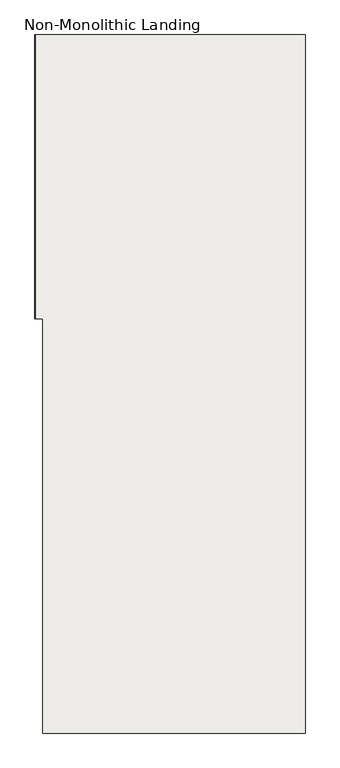
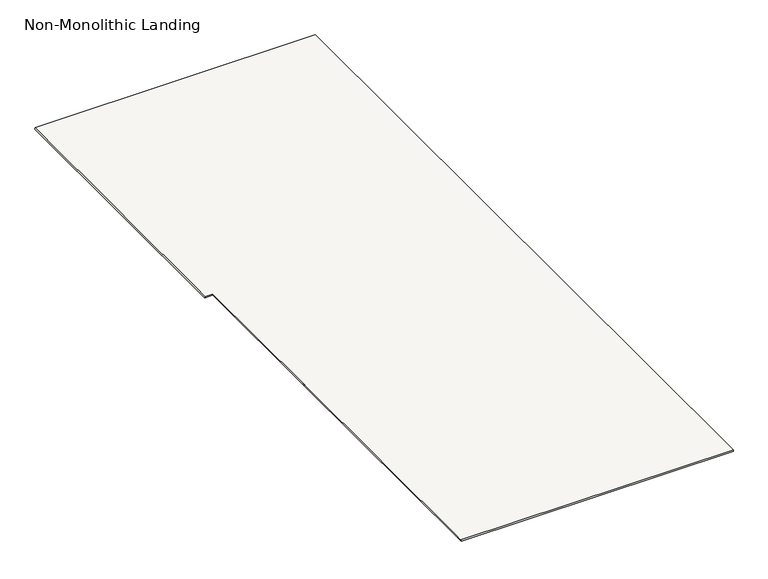
"""IFC4 building model written with IfcOpenShell, lengths in millimetres: slab geometry, Non-Monolithic Landing."""

from ifc_helpers import new_model, si_unit, origin, place, context, project, spatial, faceted_brep, source, transform, mapped, element, save


def non_monolithic_landing_c230c3b8(model_context):
    return source(origin(), model_context, "Body", "Brep", [
        faceted_brep([(16318.9400908, 13220.4345331, 26352.9411765), (16318.0900908, 13220.4345331, 26346.9411765), (16318.0900908, 12030.4345331, 26346.9411765), (16318.9400908, 12030.4345331, 26352.9411765), (16350.0, 10295.4345331, 26352.9411765), (17450.0, 10295.4345331, 26352.9411765), (17450.0, 13220.4345331, 26352.9411765), (16350.0, 13220.4345331, 26352.9411765), (16350.0, 12030.4345331, 26352.9411765), (16350.0, 11395.4345331, 26352.9411765), (17450.0, 13220.4345331, 26346.9411765), (17450.0, 10295.4345331, 26346.9411765), (16350.85, 10295.4345331, 26346.9411765), (16350.85, 11395.4345331, 26346.9411765), (16350.0, 11395.4345331, 26346.9411765), (16350.0, 12030.4345331, 26346.9411765), (16350.0, 13220.4345331, 26346.9411765)], [[[0, 1, 2, 3]], [[4, 5, 6, 7, 0, 3, 8, 9]], [[10, 11, 12, 13, 14, 15, 2, 1, 16]], [[9, 8, 15, 14]], [[0, 7, 16, 1]], [[7, 6, 10, 16]], [[6, 5, 11, 10]], [[5, 4, 12, 11]], [[13, 9, 14]], [[9, 13, 12, 4]], [[8, 3, 2, 15]]]),
    ])


if __name__ == "__main__":
    model = new_model("IFC4")
    model_context = context("Model", 3, world=origin())
    ifc_project = project(units=[si_unit("LENGTHUNIT", "METRE", prefix="MILLI")], contexts=[model_context])
    site = spatial("IfcSite", under=ifc_project)
    building = spatial("IfcBuilding", under=site)
    placement = place(None, origin())
    non_monolithic_landing_shape = non_monolithic_landing_c230c3b8(model_context)
    element("IfcSlab", 1, ObjectType="Non-Monolithic Landing", at=placement, inside=building, context=model_context, shape_type="MappedRepresentation", body=[
        mapped(non_monolithic_landing_shape, transform((0.0, 0.0, 0.0), x_axis=(1.0, 0.0, 0.0), y_axis=(0.0, 1.0, 0.0), z_axis=(0.0, 0.0, 1.0))),
    ])
    save(model, "model.ifc")

# Revit data of these elements
# Element 1 (IfcSlab, "Non-Monolithic Landing")
#   Materials on its faces: "Steel, Paint Finish, Dark Gray"
# Materials
#   "Steel, Paint Finish, Dark Gray": class "Metal", colour RGB 89 89 89, transparency 0, Description = "Steel, paint finish, dark gray, glossy", Cost = 0
